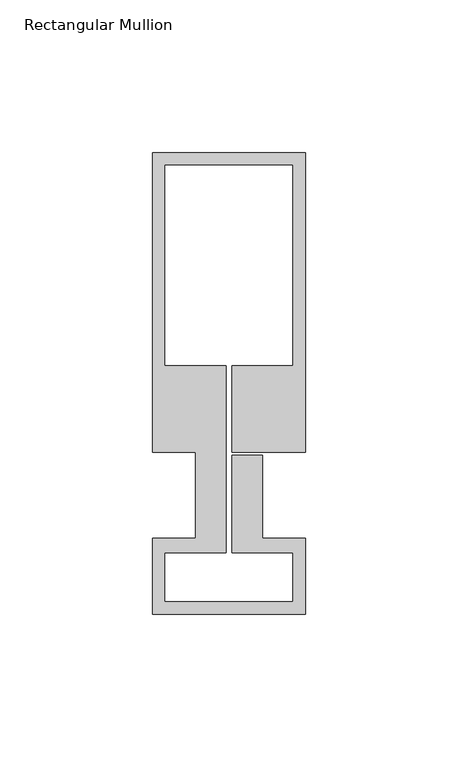
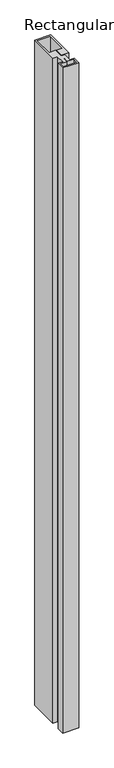
"""IFC4 building model written with IfcOpenShell, lengths in millimetres: member geometry, Rectangular Mullion : Schueco_FWS-50-HI_Mull_CovCap-20mm_Mull-85mm."""

from ifc_helpers import new_model, si_unit, frame, origin, place, context, project, spatial, polyline, outline, extrude, source, transform, mapped, element, save


def rectangular_mullion_90fada9e(model_context):
    return source(origin(), model_context, "Body", "SweptSolid", [
        extrude(outline(polyline([(-50.0, 126.0), (0.0, 126.0), (0.0, 28.0), (-24.0, 28.0), (-24.0, 56.3), (-4.0, 56.3), (-4.0, 122.0), (-46.0, 122.0), (-46.0, 56.3), (-26.0, 56.3), (-26.0, -5.0), (-46.0, -5.0), (-46.0, -21.0), (-4.0, -21.0), (-4.0, -5.0), (-24.0, -5.0), (-24.0, 27.0), (-14.0, 27.0), (-14.0, -0.1), (0.0, -0.1), (0.0, -25.0), (-50.0, -25.0), (-50.0, -0.1), (-36.0, -0.1), (-36.0, 28.0), (-50.0, 28.0), (-50.0, 126.0)])), frame((0.0, 0.0, -2200.0), z_axis=(0.0, 0.0, 1.0), x_axis=(1.0, 0.0, 0.0)), (0.0, 0.0, 1.0), 2200.0),
    ])


if __name__ == "__main__":
    model = new_model("IFC4")
    model_context = context("Model", 3, world=origin())
    ifc_project = project(units=[si_unit("LENGTHUNIT", "METRE", prefix="MILLI")], contexts=[model_context])
    site = spatial("IfcSite", under=ifc_project)
    building = spatial("IfcBuilding", under=site)
    placement = place(None, origin())
    rectangular_mullion_shape = rectangular_mullion_90fada9e(model_context)
    element("IfcMember", 1, ObjectType="Rectangular Mullion : Schueco_FWS-50-HI_Mull_CovCap-20mm_Mull-85mm", at=placement, inside=building, context=model_context, shape_type="MappedRepresentation", body=[
        mapped(rectangular_mullion_shape, transform((0.0, 0.0, 0.0), x_axis=(1.0, 0.0, 0.0), y_axis=(0.0, 1.0, 0.0), z_axis=(0.0, 0.0, 1.0))),
    ])
    save(model, "model.ifc")

# Revit data of these elements
# Type "Rectangular Mullion : Schueco_FWS-50-HI_Mull_CovCap-20mm_Mull-85mm"
#   Model = "FWS 50.HI"
#   Manufacturer = "Schueco International KG"
#   Type Comments = "Mullion"
#   Schueco thermal insulation standard = "Highly thermally insulated"
#   Burglar resistance = "RC 3"
#   Thermal insulation = "to 0.90 W/(m²K)"
#   built-in parameter 1007322 = 0.495407 (stored number, unit not read)
#   built-in parameter 1007321 = 0.0360892 (stored number, unit not read)
#   built-in parameter 1007320 = 0.0360892 (stored number, unit not read)
# Element 1 (IfcMember, "Rectangular Mullion : Schueco_FWS-50-HI_Mull_CovCap-20mm_Mull-85mm")
#   Materials on its faces: "Alu"
# Materials
#   "Alu": class "Glas", colour RGB 140 140 140, transparency 0
